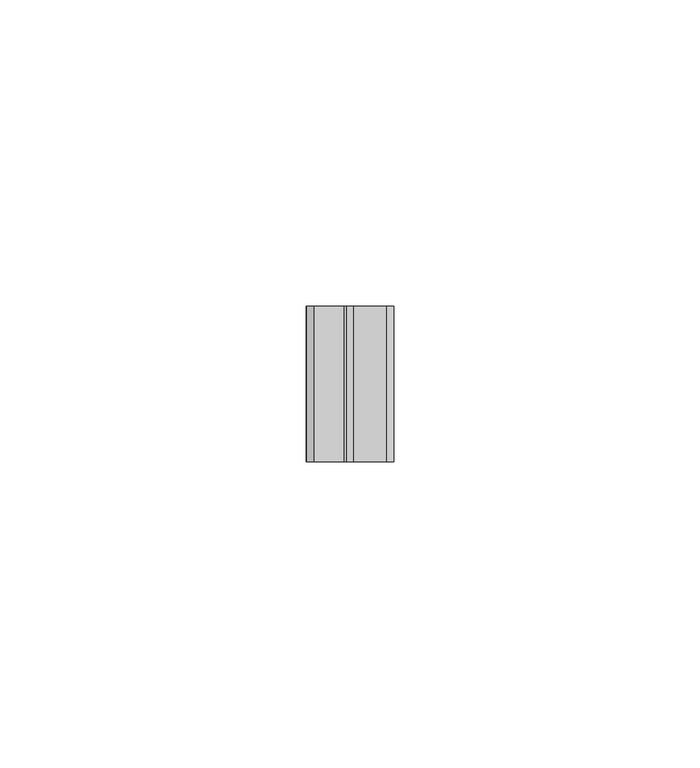
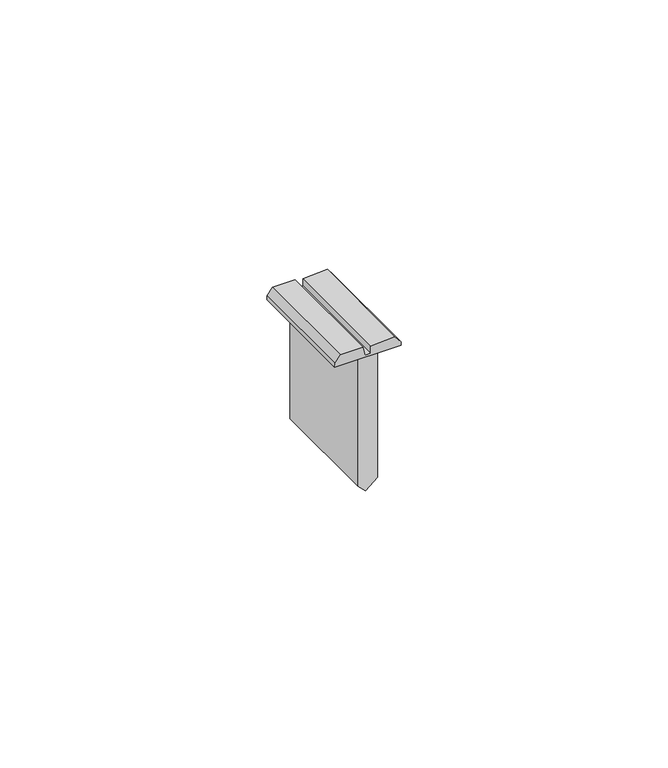
"""IFC4 building model written with IfcOpenShell, lengths in millimetres: proxy geometry, FASTENER1:FASTENER005:297402 : FASTENER1:FASTENER005:297402."""

from ifc_helpers import new_model, si_unit, frame, origin, place, context, project, spatial, polyline, outline, extrude, source, transform, mapped, element, save


def generic_models_eded0b77(model_context):
    return source(origin(), model_context, "Body", "SweptSolid", [
        extrude(outline(polyline([(42579.6987049, 10749.2762959), (42579.6987049, 10763.5726012), (42580.508527, 10763.5726012), (42582.1023984, 10762.3338991), (42581.7061629, 10757.0482169), (42580.1167322, 10757.0482169), (42580.1167322, 10755.801112), (42582.1288635, 10755.4048765), (42582.1288635, 10750.5257946), (42580.5349921, 10749.2870925), (42579.6987049, 10749.2762959)])), frame((0.0, -799.9581163, 0.0), z_axis=(0.0, 1.0, 0.0), x_axis=(0.0, 0.0, 1.0)), (0.0, 0.0, 1.0), 25.4),
        extrude(outline(polyline([(42579.6987049, 10758.526734), (42579.6987049, 10754.3198155), (42550.7399648, 10754.3198155), (42549.1244121, 10755.9768301), (42551.3049701, 10758.526734), (42579.6987049, 10758.526734)])), frame((0.0, -799.9581163, 0.0), z_axis=(0.0, 1.0, 0.0), x_axis=(0.0, 0.0, 1.0)), (0.0, 0.0, 1.0), 25.4),
    ])


if __name__ == "__main__":
    model = new_model("IFC4")
    model_context = context("Model", 3, world=origin())
    ifc_project = project(units=[si_unit("LENGTHUNIT", "METRE", prefix="MILLI")], contexts=[model_context])
    site = spatial("IfcSite", under=ifc_project)
    building = spatial("IfcBuilding", under=site)
    placement = place(None, origin())
    generic_models_shape = generic_models_eded0b77(model_context)
    element("IfcBuildingElementProxy", 1, Name="FASTENER1:FASTENER005:297402 : FASTENER1:FASTENER005:297402", ObjectType="FASTENER1:FASTENER005:297402 : FASTENER1:FASTENER005:297402", at=placement, inside=building, context=model_context, shape_type="MappedRepresentation", body=[
        mapped(generic_models_shape, transform((0.0, 0.0, 0.0), x_axis=(1.0, 0.0, 0.0), y_axis=(0.0, 1.0, 0.0), z_axis=(0.0, 0.0, 1.0))),
    ])
    save(model, "model.ifc")

# Revit data of these elements
# Type "FASTENER1:FASTENER005:297402 : FASTENER1:FASTENER005:297402"
#   NameOverride = "FASTENER1:FASTENER005:297402"
#   ObjectTypeOverride = "FASTENER1:FASTENER005"
#   Reference = "FASTENER005"
#   Category = "Generic Models"
#   Tag = "297402"
# Element 1 (IfcBuildingElementProxy, "FASTENER1:FASTENER005:297402 : FASTENER1:FASTENER005:297402")
#   Materials on its faces: "ENGINEERED PANCAKE HEAD FASTENER @ 12\" O.C."
# Materials
#   "ENGINEERED PANCAKE HEAD FASTENER @ 12\" O.C.": class "Unassigned", colour RGB 255 255 255, transparency 0, Cost = 0
